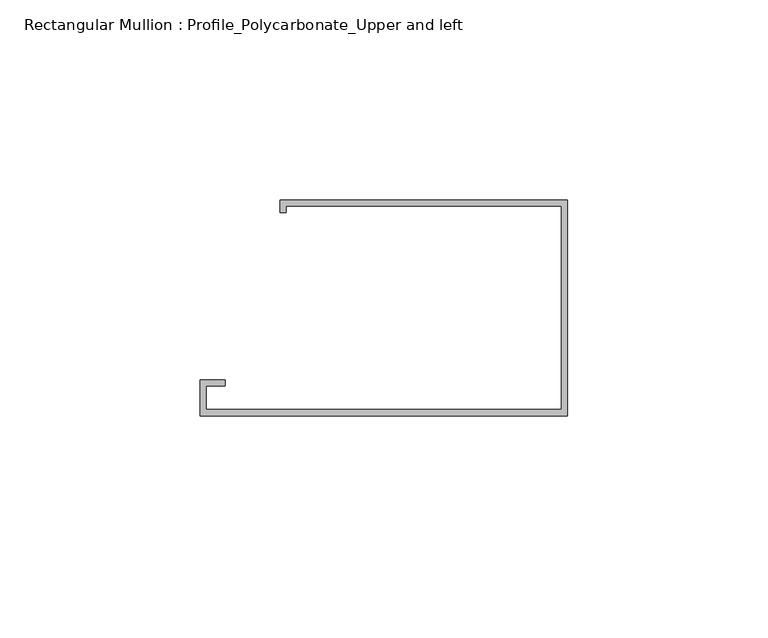
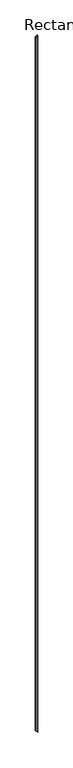
"""IFC4 building model written with IfcOpenShell, lengths in millimetres: member geometry, Rectangular Mullion : Profile_Polycarbonate_Upper and left."""

from ifc_helpers import new_model, si_unit, origin, place, context, project, spatial, faceted_brep, source, transform, mapped, element, save


def rectangular_mullion_profile_polycarbonate_upper_and_left_f00f8bbb(model_context):
    return source(origin(), model_context, "Body", "Brep", [
        faceted_brep([(0.0, 25.015825, 0.0), (0.0, -28.984575, 0.0), (0.0, -28.984575, -31744.2078079), (0.0, 25.015825, -31744.2078079), (-71.9836, 25.015825, -69.046742), (-71.9836, 25.015825, -31669.1624326), (-71.9836, 21.840825, -69.046742), (-71.9836, 21.840825, -31669.1624326), (-70.3961, 21.840825, -67.5240104), (-70.3961, 21.840825, -31670.8174559), (-70.3961, 23.428325, -67.5240104), (-70.3961, 23.428325, -31670.8174559), (-1.5875, 23.428325, -1.5227316), (-1.5875, 23.428325, -31742.5527846), (-1.5875, -27.397075, -1.5227316), (-1.5875, -27.397075, -31742.5527846), (-90.4113, -27.397075, -86.7226105), (-90.4113, -27.397075, -31649.9509224), (-90.4113, -21.580475, -86.7226105), (-90.4113, -21.580475, -31649.9509224), (-85.6488, -21.580475, -82.1544157), (-85.6488, -21.580475, -31654.9159922), (-85.6488, -19.992975, -82.1544157), (-85.6488, -19.992975, -31654.9159922), (-91.9988, -19.992975, -88.2453421), (-91.9988, -19.992975, -31648.2958991), (-91.9988, -28.984575, -88.2453421), (-91.9988, -28.984575, -31648.2958991)], [[[0, 1, 2, 3]], [[4, 0, 3, 5]], [[6, 4, 5, 7]], [[8, 6, 7, 9]], [[10, 8, 9, 11]], [[12, 10, 11, 13]], [[14, 12, 13, 15]], [[16, 14, 15, 17]], [[18, 16, 17, 19]], [[20, 18, 19, 21]], [[22, 20, 21, 23]], [[24, 22, 23, 25]], [[26, 24, 25, 27]], [[1, 26, 27, 2]], [[1, 0, 4, 6, 8, 10, 12, 14, 16, 18, 20, 22, 24, 26]], [[2, 27, 25, 23, 21, 19, 17, 15, 13, 11, 9, 7, 5, 3]]]),
    ])


if __name__ == "__main__":
    model = new_model("IFC4")
    model_context = context("Model", 3, world=origin())
    ifc_project = project(units=[si_unit("LENGTHUNIT", "METRE", prefix="MILLI")], contexts=[model_context])
    site = spatial("IfcSite", under=ifc_project)
    building = spatial("IfcBuilding", under=site)
    placement = place(None, origin())
    rectangular_mullion_profile_polycarbonate_upper_and_left_shape = rectangular_mullion_profile_polycarbonate_upper_and_left_f00f8bbb(model_context)
    element("IfcMember", 1, ObjectType="Rectangular Mullion : Profile_Polycarbonate_Upper and left", at=placement, inside=building, context=model_context, shape_type="MappedRepresentation", body=[
        mapped(rectangular_mullion_profile_polycarbonate_upper_and_left_shape, transform((0.0, 0.0, 0.0), x_axis=(1.0, 0.0, 0.0), y_axis=(0.0, 1.0, 0.0), z_axis=(0.0, 0.0, 1.0))),
    ])
    save(model, "model.ifc")

# Revit data of these elements
# Type "Rectangular Mullion : Profile_Polycarbonate_Upper and left"
#   built-in parameter 1007322 = 0.177167 (stored number, unit not read)
#   built-in parameter 1007321 = 0.00520833 (stored number, unit not read)
#   built-in parameter 1007320 = 0 (stored number, unit not read)
